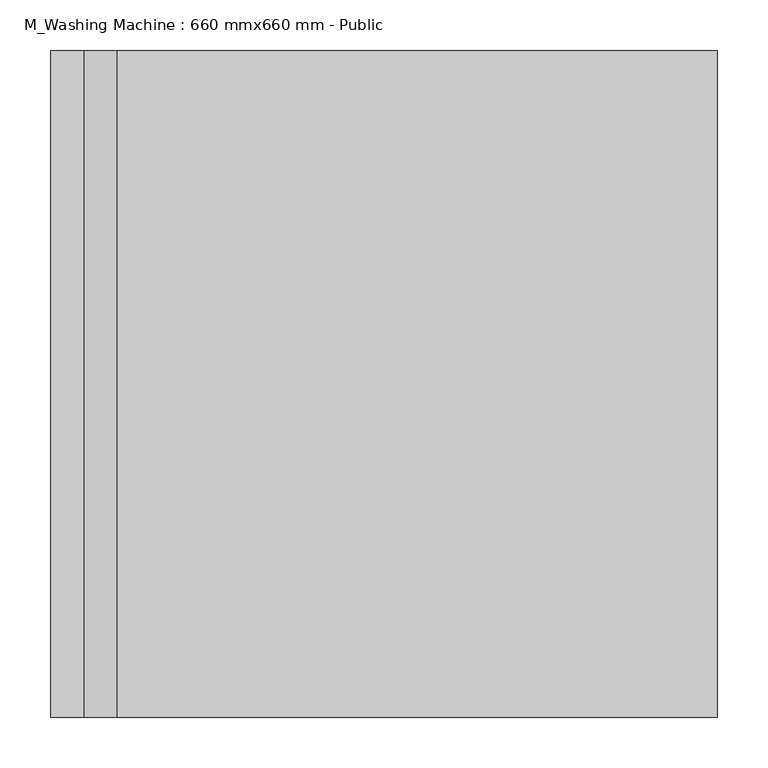
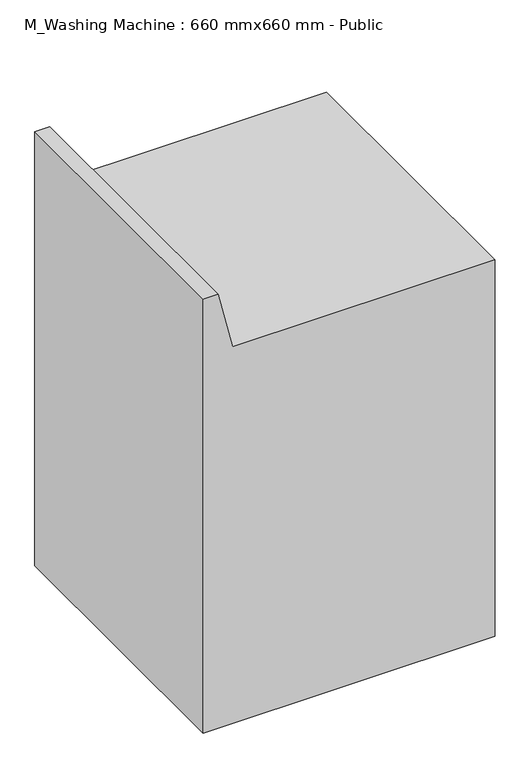
"""IFC4 building model written with IfcOpenShell, lengths in millimetres: flow terminal geometry, M_Washing Machine : 660 mmx660 mm - Public."""

from ifc_helpers import new_model, si_unit, frame, origin, place, context, project, spatial, polyline, outline, extrude, source, transform, mapped, element, save


def m_washing_machine_660_mmx660_mm_public_59181b66(model_context):
    return source(origin(), model_context, "Body", "SweptSolid", [
        extrude(outline(polyline([(0.0, 660.0), (900.0, 660.0), (900.0, 65.88125), (1037.31875, 33.3375), (1037.31875, 0.0), (0.0, 0.0), (0.0, 660.0)])), frame((0.0, -330.0, 0.0), z_axis=(0.0, 1.0, 0.0), x_axis=(0.0, 0.0, 1.0)), (0.0, 0.0, 1.0), 660.0),
    ])


if __name__ == "__main__":
    model = new_model("IFC4")
    model_context = context("Model", 3, world=origin())
    ifc_project = project(units=[si_unit("LENGTHUNIT", "METRE", prefix="MILLI")], contexts=[model_context])
    site = spatial("IfcSite", under=ifc_project)
    building = spatial("IfcBuilding", under=site)
    placement = place(None, origin())
    m_washing_machine_660_mmx660_mm_public_shape = m_washing_machine_660_mmx660_mm_public_59181b66(model_context)
    element("IfcFlowTerminal", 1, ObjectType="M_Washing Machine : 660 mmx660 mm - Public", at=placement, inside=building, context=model_context, shape_type="MappedRepresentation", body=[
        mapped(m_washing_machine_660_mmx660_mm_public_shape, transform((0.0, 0.0, 0.0), x_axis=(1.0, 0.0, 0.0), y_axis=(0.0, 1.0, 0.0), z_axis=(0.0, 0.0, 1.0))),
    ])
    save(model, "model.ifc")

# Revit data of these elements
# Type "M_Washing Machine : 660 mmx660 mm - Public"
#   Sanitary Radius = 25 mm
#   Sanitary Diameter = 50 mm
#   Washing Machine Width = 660 mm
#   Washing Machine Length = 660 mm
#   Washing Machine Height = 900 mm
#   WFU = 3
#   Voltage = 120 V
#   Hot Water Radius = 12.5 mm
#   Hot Water Diameter = 25 mm
#   Half Washing Machine Width = 330 mm
#   HWFU = 2.25
#   Flow Pressure [instance default] = 55158.0 Pa
#   Cold Water Radius = 12.5 mm
#   Cold Water Diameter = 25 mm
#   CWFU = 2.25
#   Apparent Load = 600 VA
#   Number of Poles = 1
#   Washing Machine Material = none
#   Load Classification = Electric Clothes Dryer
#   Default Elevation = 0
